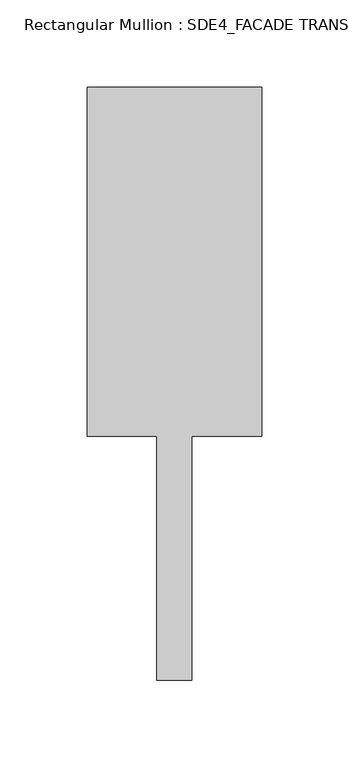
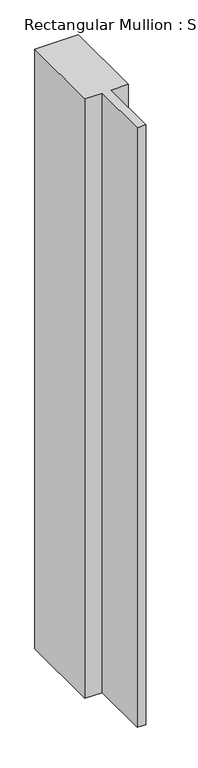
"""IFC4 building model written with IfcOpenShell, lengths in millimetres: member geometry, Rectangular Mullion : SDE4_FACADE TRANSOM TYPE 1."""

from ifc_helpers import new_model, si_unit, frame, origin, place, context, project, spatial, polyline, outline, extrude, source, transform, mapped, element, save


def rectangular_mullion_sde4_facade_transom_type_1_13196fc2(model_context):
    return source(origin(), model_context, "Body", "SweptSolid", [
        extrude(outline(polyline([(50.0, 132.5), (50.0, -67.5), (10.0, -67.5), (10.0, -207.5), (-10.0, -207.5), (-10.0, -67.5), (-50.0, -67.5), (-50.0, 132.5), (50.0, 132.5)])), frame((0.0, 0.0, -1466.5), z_axis=(0.0, 0.0, 1.0), x_axis=(1.0, 0.0, 0.0)), (0.0, 0.0, 1.0), 1466.5),
    ])


if __name__ == "__main__":
    model = new_model("IFC4")
    model_context = context("Model", 3, world=origin())
    ifc_project = project(units=[si_unit("LENGTHUNIT", "METRE", prefix="MILLI")], contexts=[model_context])
    site = spatial("IfcSite", under=ifc_project)
    building = spatial("IfcBuilding", under=site)
    placement = place(None, origin())
    rectangular_mullion_sde4_facade_transom_type_1_shape = rectangular_mullion_sde4_facade_transom_type_1_13196fc2(model_context)
    element("IfcMember", 1, ObjectType="Rectangular Mullion : SDE4_FACADE TRANSOM TYPE 1", at=placement, inside=building, context=model_context, shape_type="MappedRepresentation", body=[
        mapped(rectangular_mullion_sde4_facade_transom_type_1_shape, transform((0.0, 0.0, 0.0), x_axis=(1.0, 0.0, 0.0), y_axis=(0.0, 1.0, 0.0), z_axis=(0.0, 0.0, 1.0))),
    ])
    save(model, "model.ifc")

# Revit data of these elements
# Type "Rectangular Mullion : SDE4_FACADE TRANSOM TYPE 1"
#   built-in parameter 1007322 = 1.11549 (stored number, unit not read)
#   built-in parameter 1007321 = 0.164042 (stored number, unit not read)
#   built-in parameter 1007320 = 0.164042 (stored number, unit not read)
